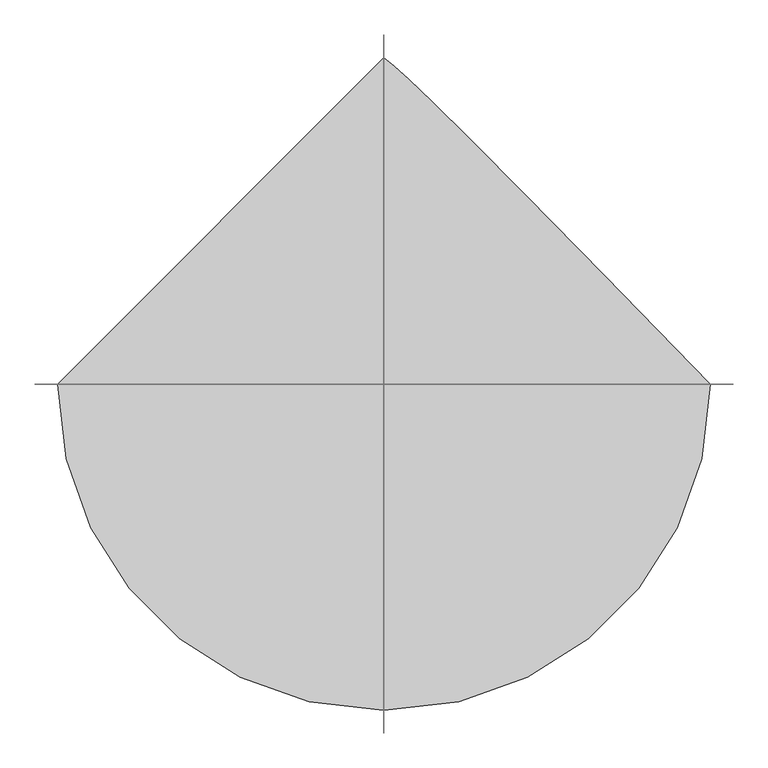
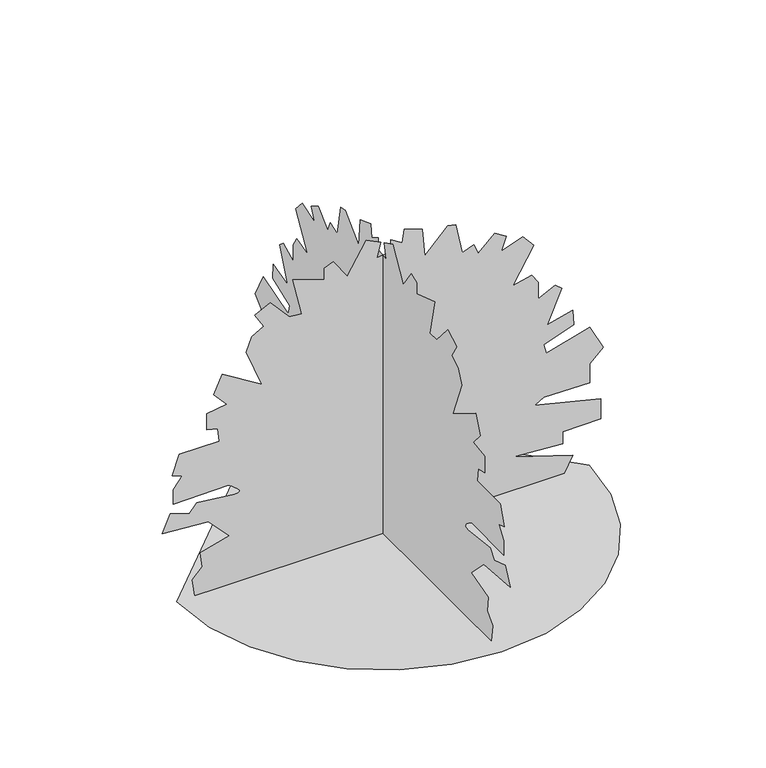
"""IFC4 building model written with IfcOpenShell, lengths in millimetres: proxy geometry, privet 26761 : privet 26761."""

import ifcopenshell
import ifcopenshell.guid

model = None  # the IFC model being written
_history = None  # IfcOwnerHistory: only IFC2X3 demands one
_inside = {}  # id of a spatial element -> (the spatial element, [elements in it])
_under = {}  # id of a project, library or spatial element -> (it, [spatial elements below it])
_declared = {}  # id of a project -> (the project, [libraries it declares])
_typed = {}  # id of a type object -> (the type object, [elements of that type])
_made_of = {}  # id of a material, layer set ... -> (it, [elements and type objects made of it])


def new_model(schema):
    """Start an empty IFC model of exactly this schema.

    Asked for "IFC4X3", IfcOpenShell would pick the latest addendum, in which some entities
    have other attributes; the version numbers below select the first issue.
    IFC2X3 requires an IfcOwnerHistory on every rooted entity: one is made here for all.
    """
    global model, _history
    if schema == "IFC4X3":
        model = ifcopenshell.file(schema_version=(4, 3, 0, 0))
    else:
        model = ifcopenshell.file(schema=schema)
    _inside.clear()
    _under.clear()
    _declared.clear()
    _typed.clear()
    _made_of.clear()
    _history = None
    if model.schema == "IFC2X3":
        org = make("IfcOrganization", Name="unknown")
        user = make(
            "IfcPersonAndOrganization",
            ThePerson=make("IfcPerson", FamilyName="unknown"),
            TheOrganization=org,
        )
        app = make(
            "IfcApplication",
            ApplicationDeveloper=org,
            Version="unknown",
            ApplicationFullName="unknown",
            ApplicationIdentifier="unknown",
        )
        _history = make(
            "IfcOwnerHistory",
            OwningUser=user,
            OwningApplication=app,
            ChangeAction="ADDED",
            CreationDate=0,
        )
    return model


def make(cls, **values):
    """One entity of the class cls with the attributes given. An attribute that is None is left unset."""
    return model.create_entity(
        cls, **{name: value for name, value in values.items() if value is not None}
    )


def rooted(cls, **values):
    """An entity with a GlobalId (a new one), such as an element, a storey or a relation."""
    return make(cls, GlobalId=ifcopenshell.guid.new(), OwnerHistory=_history, **values)


def si_unit(unit_type, name, prefix=None):
    """IfcSIUnit, for example si_unit("LENGTHUNIT", "METRE", prefix="MILLI")."""
    return make("IfcSIUnit", UnitType=unit_type, Prefix=prefix, Name=name)


def assignment(units):
    """IfcUnitAssignment: the units of a project."""
    return None if units is None else make("IfcUnitAssignment", Units=units)


def point(xyz):
    """IfcCartesianPoint."""
    return None if xyz is None else make("IfcCartesianPoint", Coordinates=xyz)


def direction(xyz):
    """IfcDirection."""
    return None if xyz is None else make("IfcDirection", DirectionRatios=xyz)


def frame(location, z_axis=None, x_axis=None):
    """IfcAxis2Placement3D, a coordinate frame: its origin and axes. An axis left out is left unset."""
    return make(
        "IfcAxis2Placement3D",
        Location=point(location),
        Axis=direction(z_axis),
        RefDirection=direction(x_axis),
    )


def origin():
    """The frame at (0, 0, 0) with its axes left unset."""
    return frame((0.0, 0.0, 0.0))


def place(relative_to, where):
    """IfcLocalPlacement: puts the frame where relative to a parent placement (None: the world)."""
    return make(
        "IfcLocalPlacement", PlacementRelTo=relative_to, RelativePlacement=where
    )


def context(
    kind, dimensions, precision=None, world=None, true_north=None, identifier=None
):
    """IfcGeometricRepresentationContext, for example the 3D "Model" context."""
    return make(
        "IfcGeometricRepresentationContext",
        ContextIdentifier=identifier,
        ContextType=kind,
        CoordinateSpaceDimension=dimensions,
        Precision=precision,
        WorldCoordinateSystem=world,
        TrueNorth=true_north,
    )


def project(units=None, contexts=None):
    """IfcProject with its units and contexts."""
    return rooted(
        "IfcProject",
        Name="project",
        RepresentationContexts=contexts,
        UnitsInContext=assignment(units),
    )


def spatial(cls, under=None, at=None, **own):
    """A site, building, storey or space (cls), placed at a placement, below another one or the project."""
    s = rooted(cls, ObjectPlacement=at, **own)
    if under is not None:
        _under.setdefault(under.id(), (under, []))[1].append(s)
    return s


def point_list(points):
    """IfcCartesianPointList2D or 3D."""
    cls = (
        "IfcCartesianPointList2D" if len(points[0]) == 2 else "IfcCartesianPointList3D"
    )
    return make(cls, CoordList=points)


def triangles(points, corners, closed=None, point_numbers=None):
    """IfcTriangulatedFaceSet: each triangle names its three corners, points numbered from 1."""
    return make(
        "IfcTriangulatedFaceSet",
        Coordinates=point_list(points),
        Closed=closed,
        CoordIndex=corners,
        PnIndex=point_numbers,
    )


def shape(context_of_items, identifier, shape_type, items):
    """IfcShapeRepresentation: the items that make up one representation, for example the "Body"."""
    return make(
        "IfcShapeRepresentation",
        ContextOfItems=context_of_items,
        RepresentationIdentifier=identifier,
        RepresentationType=shape_type,
        Items=items,
    )


def source(mapping_origin, context_of_items, identifier, shape_type, items):
    """IfcRepresentationMap: a shape defined once, which mapped items show again and again."""
    return make(
        "IfcRepresentationMap",
        MappingOrigin=mapping_origin,
        MappedRepresentation=shape(context_of_items, identifier, shape_type, items),
    )


def transform(
    local_origin,
    x_axis=None,
    y_axis=None,
    z_axis=None,
    scale=None,
    scale2=None,
    scale3=None,
    uniform=True,
):
    """IfcCartesianTransformationOperator3D, or its non-uniform kind. x_axis, y_axis, z_axis: its Axis1, 2, 3."""
    if uniform:
        return make(
            "IfcCartesianTransformationOperator3D",
            Axis1=direction(x_axis),
            Axis2=direction(y_axis),
            LocalOrigin=point(local_origin),
            Scale=scale,
            Axis3=direction(z_axis),
        )
    return make(
        "IfcCartesianTransformationOperator3DnonUniform",
        Axis1=direction(x_axis),
        Axis2=direction(y_axis),
        LocalOrigin=point(local_origin),
        Scale=scale,
        Axis3=direction(z_axis),
        Scale2=scale2,
        Scale3=scale3,
    )


def mapped(mapping_source, mapping_target):
    """IfcMappedItem: shows the shape of a source again, moved by a transform."""
    return make(
        "IfcMappedItem", MappingSource=mapping_source, MappingTarget=mapping_target
    )


def made_of(thing, what):
    """Note that an element or type object is made of a material, layer set ...; save() writes the relation."""
    if what is not None:
        _made_of.setdefault(what.id(), (what, []))[1].append(thing)
    return thing


def element(
    cls,
    number,
    at=None,
    inside=None,
    cuts=None,
    type_object=None,
    material=None,
    context=None,
    identifier="Body",
    shape_type=None,
    held_by="IfcProductDefinitionShape",
    body=None,
    shapes=None,
    **own,
):
    """One element of the class cls, such as IfcWall. Its Tag is "e" and its number.

    at: its placement. inside: the storey or other place that contains it. cuts: it is an
    opening in that element (IfcRelVoidsElement). A single representation is given by context,
    identifier, shape_type and body (its items); several are given by shapes. held_by: the class
    of the entity that holds the representations. save() writes the other relations.
    """
    e = rooted(cls, Tag="e%d" % number, ObjectPlacement=at, **own)
    if body is not None:
        shapes = [shape(context, identifier, shape_type, body)]
    if shapes is not None:
        e.Representation = make(held_by, Representations=shapes)
    if inside is not None:
        _inside.setdefault(inside.id(), (inside, []))[1].append(e)
    if cuts is not None:
        rooted(
            "IfcRelVoidsElement", RelatingBuildingElement=cuts, RelatedOpeningElement=e
        )
    if type_object is not None:
        _typed.setdefault(type_object.id(), (type_object, []))[1].append(e)
    return made_of(e, material)


def aggregate(whole, parts):
    """IfcRelAggregates: a whole, such as a stair, and the parts it consists of."""
    return rooted("IfcRelAggregates", RelatingObject=whole, RelatedObjects=parts)


def save(model, path):
    """Write the relations noted so far, then the file.

    IfcRelAggregates (storeys below a building ...), IfcRelContainedInSpatialStructure (elements
    in a storey), IfcRelDefinesByType, IfcRelAssociatesMaterial and IfcRelDeclares: one each for
    every whole, place, type object, material and project.
    """
    for whole, parts in _under.values():
        aggregate(whole, parts)
    for where, things in _inside.values():
        rooted(
            "IfcRelContainedInSpatialStructure",
            RelatedElements=things,
            RelatingStructure=where,
        )
    for kind, things in _typed.values():
        rooted("IfcRelDefinesByType", RelatedObjects=things, RelatingType=kind)
    for what, things in _made_of.values():
        rooted("IfcRelAssociatesMaterial", RelatedObjects=things, RelatingMaterial=what)
    for by, libraries in _declared.values():
        rooted("IfcRelDeclares", RelatingContext=by, RelatedDefinitions=libraries)
    model.write(path)


def entourage_76426c84(model_context):
    return source(origin(), model_context, "Body", "Tessellation", [
        triangles([(-629.6484856, 0.0, 4.95e-05), (-613.003862, -144.2738427, 4.95e-05), (-565.5947282, -276.766137, 4.95e-05), (-491.2235046, -393.6824018, 4.95e-05), (-393.6824018, -491.2235046, 4.95e-05), (-276.766137, -565.5947282, 4.95e-05), (-144.2738427, -613.003862, 4.95e-05), (2.75e-05, -629.6484856, 4.95e-05), (144.2738427, -613.003862, 4.95e-05), (276.766137, -565.5947282, 4.95e-05), (393.6824018, -491.2235046, 4.95e-05), (491.2235046, -393.6824018, 4.95e-05), (565.5947282, -276.766137, 4.95e-05), (613.003862, -144.2738427, 4.95e-05), (629.6484856, 5.5e-05, 4.95e-05), (425.0259828, 209.8919668, 4.95e-05), (273.329519, 364.4266657, 4.95e-05), (165.7386299, 472.8288062, 4.95e-05), (93.4306343, 544.3247692, 4.95e-05), (47.5853949, 588.1448779, 4.95e-05), (19.3822403, 613.5093544, 4.95e-05), (-8.26e-05, 629.6484856, 4.95e-05), (-2.3e-06, -573.7887774, 0.0), (-2.3e-06, -582.0844193, 55.3049682), (-2.3e-06, -551.6679256, 85.7227472), (-2.3e-06, -557.1974936, 132.7320781), (0.0, -468.7089269, 157.747784), (0.0, -532.310568, 224.1137004), (0.0, -673.33906, 235.174635), (0.0, -648.4495909, 290.4795987), (0.0, -590.3800612, 271.1222591), (0.0, -568.2592094, 298.7752406), (0.0, -452.1176431, 284.9500125), (0.0, -441.363285, 285.9964966), (0.0, -436.849716, 288.9327454), (0.0, -437.5355026, 293.4387022), (0.0, -442.379284, 299.2019587), (0.0, -450.3447135, 305.9101067), (0.0, -460.3904303, 313.2456327), (0.0, -471.4750008, 320.898654), (0.0, -640.153949, 318.1325801), (0.0, -640.153949, 365.1403939), (0.0, -612.5034565, 401.0890354), (0.0, -642.9199865, 412.1507512), (0.0, -620.7990984, 472.9863184), (0.0, -499.1280004, 472.9863184), (0.0, -504.6575684, 514.4645279), (0.0, -537.840136, 522.7601698), (0.0, -537.840136, 575.3000951), (0.0, -477.0045688, 583.595737), (0.0, -515.7192842, 627.8400204), (0.0, -490.8323585, 685.9095137), (0.0, -369.1612241, 611.2487366), (0.0, -416.1690016, 730.1537607), (0.0, -399.5777178, 774.3980804), (0.0, -363.6291126, 796.521512), (0.0, -391.2820759, 840.7632156), (0.0, -344.2742984, 865.6526848), (0.0, -286.2022435, 799.2850061), (0.0, -247.4898354, 796.521512), (0.0, -275.1430711, 915.4265362), (0.0, -178.3586263, 882.2439686), (0.0, -178.3586263, 918.190103), (0.0, -150.7061354, 929.2517824), (0.0, -109.2271628, 868.4161789), (0.0, -51.1571472, 965.2003876), (0.0, -6.9130699, 943.0795721), (0.0, -17.9741141, 896.0692148), (0.0, 23.5046359, 901.5988192), (0.0, 23.5046359, 940.3134619), (0.0, 59.4527891, 918.190103), (0.0, 64.9833881, 959.6708559), (0.0, 120.2883518, 940.3134619), (0.0, 128.5842571, 851.8248951), (0.0, 197.7154571, 923.7221781), (0.0, 222.6026553, 918.190103), (0.0, 241.9594862, 821.4084377), (0.0, 277.9066016, 835.2336113), (0.0, 291.7343731, 802.0510437), (0.0, 341.5082245, 849.0588575), (0.0, 377.456866, 826.9379694), (0.0, 360.8655822, 785.4597599), (0.0, 427.2307174, 807.580648), (0.0, 460.413285, 768.8684761), (0.0, 396.8142237, 661.022588), (0.0, 454.883717, 674.8503777), (0.0, 474.2410747, 644.4313042), (0.0, 474.2410747, 591.8913789), (0.0, 526.7809999, 616.7782682), (0.0, 546.1357779, 600.1870208), (0.0, 501.8915308, 497.8732441), (0.0, 579.3183818, 517.2305655), (0.0, 582.0844193, 470.2202445), (0.0, 490.8323585, 437.0376769), (0.0, 499.1280004, 406.6211469), (0.0, 631.8583071, 445.3333188), (0.0, 673.33906, 365.1403939), (0.0, 631.8583071, 326.428222), (0.0, 631.8583071, 265.592673), (0.0, 490.8323585, 268.3587287), (0.0, 463.1793589, 251.7661732), (0.0, 665.0434181, 201.9918131), (0.0, 665.0434181, 138.3909441), (0.0, 548.9018517, 135.6256423), (0.0, 548.9018517, 96.9122169), (0.0, 399.5777178, 107.9731605), (0.0, 579.3183818, 49.9031495), (0.0, 554.4314198, 0.1285451), (-573.7887774, 9.96e-05, 4.86e-05), (-582.0844193, 9.63e-05, 55.3049682), (-551.6679256, 9.44e-05, 85.7227472), (-557.1974936, 9.16e-05, 132.7320781), (-468.7089269, 8.79e-05, 157.747784), (-532.310568, 8.39e-05, 224.1137004), (-673.33906, 8.33e-05, 235.174635), (-648.4495909, 8e-05, 290.4795987), (-590.3800612, 8.11e-05, 271.1222591), (-568.2592094, 7.95e-05, 298.7752406), (-452.1176431, 8.03e-05, 284.9500125), (-441.363285, 8.02e-05, 285.9964966), (-436.849716, 8.01e-05, 288.9327454), (-437.5355026, 7.98e-05, 293.4387022), (-442.379284, 7.95e-05, 299.2019587), (-450.3447135, 7.91e-05, 305.9101067), (-460.3904303, 7.86e-05, 313.2456327), (-471.4750008, 7.82e-05, 320.898654), (-640.153949, 7.83e-05, 318.1325801), (-640.153949, 7.55e-05, 365.1403939), (-612.5034565, 7.34e-05, 401.0890354), (-642.9199865, 7.27e-05, 412.1507512), (-620.7990984, 6.91e-05, 472.9863184), (-499.1280004, 6.91e-05, 472.9863184), (-504.6575684, 6.66e-05, 514.4645279), (-537.840136, 6.61e-05, 522.7601698), (-537.840136, 6.3e-05, 575.3000951), (-477.0045688, 6.25e-05, 583.595737), (-515.7192842, 5.99e-05, 627.8400204), (-490.8323585, 5.64e-05, 685.9095137), (-369.1612241, 6.09e-05, 611.2487366), (-416.1690016, 5.38e-05, 730.1537607), (-399.5777178, 5.11e-05, 774.3980804), (-363.6291126, 4.98e-05, 796.521512), (-391.2820759, 4.72e-05, 840.7632156), (-344.2742984, 4.57e-05, 865.6526848), (-286.2022435, 4.96e-05, 799.2850061), (-247.4898354, 4.98e-05, 796.521512), (-275.1430711, 4.27e-05, 915.4265362), (-178.3586263, 4.47e-05, 882.2439686), (-178.3586263, 4.26e-05, 918.190103), (-150.7061354, 4.19e-05, 929.2517824), (-109.2274081, 4.55e-05, 868.4161789), (-51.1571472, 3.98e-05, 965.2003876), (-6.9131466, 4.11e-05, 943.0795721), (-17.9741902, 4.39e-05, 896.0692148), (23.5045859, 4.35e-05, 901.5988192), (23.5045859, 4.12e-05, 940.3134619), (59.4527891, 4.26e-05, 918.190103), (64.9833881, 4.01e-05, 959.6708559), (120.2883518, 4.12e-05, 940.3134619), (128.5840028, 4.65e-05, 851.8248951), (197.7152028, 4.22e-05, 923.7221781), (222.6026553, 4.26e-05, 918.190103), (241.9592318, 4.83e-05, 821.4084377), (277.9066016, 4.75e-05, 835.2336113), (291.7343731, 4.95e-05, 802.0510437), (341.5082245, 4.67e-05, 849.0588575), (377.456866, 4.8e-05, 826.9379694), (360.8655822, 5.05e-05, 785.4597599), (427.2307174, 4.92e-05, 807.580648), (460.413285, 5.15e-05, 768.8684761), (396.8142237, 5.79e-05, 661.022588), (454.883717, 5.71e-05, 674.8503777), (474.2410747, 5.89e-05, 644.4313042), (474.2410747, 6.2e-05, 591.8913789), (526.7809999, 6.05e-05, 616.7782682), (546.1357779, 6.15e-05, 600.1870208), (501.8915308, 6.76e-05, 497.8732441), (579.3183818, 6.65e-05, 517.2305655), (582.0844193, 6.93e-05, 470.2202445), (490.8323585, 7.12e-05, 437.0376769), (499.1280004, 7.31e-05, 406.6211469), (631.8583071, 7.07e-05, 445.3333188), (673.33906, 7.55e-05, 365.1403939), (631.8583071, 7.78e-05, 326.428222), (631.8583071, 8.15e-05, 265.592673), (490.8323585, 8.13e-05, 268.3587287), (463.1793589, 8.23e-05, 251.7661732), (665.0434181, 8.52e-05, 201.9918131), (665.0434181, 8.9e-05, 138.3909441), (548.9018517, 8.92e-05, 135.6258967), (548.9018517, 9.15e-05, 96.9122169), (399.5777178, 9.09e-05, 107.9734149), (579.3183818, 9.43e-05, 49.9031495), (554.4314198, 9.73e-05, 0.1285937)], [[21, 22, 1], [20, 21, 1], [19, 20, 1], [18, 19, 1], [17, 18, 1], [17, 1, 2], [17, 2, 3], [17, 3, 4], [16, 17, 4], [16, 4, 5], [16, 5, 6], [16, 6, 7], [16, 7, 8], [16, 8, 9], [16, 9, 10], [16, 10, 11], [16, 11, 12], [15, 16, 12], [14, 15, 12], [13, 14, 12], [60, 61, 62], [69, 70, 71], [28, 29, 30], [28, 30, 31], [71, 72, 73], [71, 73, 74], [91, 92, 93], [91, 93, 94], [106, 107, 108], [106, 108, 23], [51, 52, 53], [50, 51, 53], [104, 105, 106], [56, 57, 58], [56, 58, 59], [98, 99, 100], [40, 41, 42], [40, 42, 43], [43, 44, 45], [43, 45, 46], [40, 43, 46], [28, 31, 32], [102, 103, 104], [101, 102, 104], [101, 104, 106], [77, 78, 79], [106, 23, 24], [106, 24, 25], [65, 66, 67], [65, 67, 68], [106, 25, 26], [106, 26, 27], [48, 49, 50], [47, 48, 50], [80, 81, 82], [79, 80, 82], [95, 96, 97], [95, 97, 98], [95, 98, 100], [63, 64, 65], [62, 63, 65], [89, 90, 91], [88, 89, 91], [27, 28, 32], [27, 32, 33], [106, 27, 33], [106, 33, 34], [106, 34, 35], [101, 106, 35], [101, 35, 36], [83, 84, 85], [82, 83, 85], [85, 86, 87], [85, 87, 88], [69, 71, 74], [75, 76, 77], [74, 75, 77], [60, 62, 65], [79, 82, 85], [95, 100, 101], [95, 101, 36], [94, 95, 36], [91, 94, 36], [88, 91, 36], [85, 88, 36], [79, 85, 36], [77, 79, 36], [74, 77, 36], [69, 74, 36], [68, 69, 36], [65, 68, 36], [60, 65, 36], [60, 36, 37], [60, 37, 38], [59, 60, 38], [59, 38, 39], [59, 39, 40], [47, 50, 53], [46, 47, 53], [40, 46, 53], [59, 40, 53], [59, 53, 54], [56, 59, 54], [56, 54, 55], [146, 147, 148], [155, 156, 157], [114, 115, 116], [114, 116, 117], [157, 158, 159], [157, 159, 160], [177, 178, 179], [177, 179, 180], [192, 193, 194], [192, 194, 109], [137, 138, 139], [136, 137, 139], [190, 191, 192], [142, 143, 144], [142, 144, 145], [184, 185, 186], [126, 127, 128], [126, 128, 129], [129, 130, 131], [129, 131, 132], [126, 129, 132], [114, 117, 118], [188, 189, 190], [187, 188, 190], [187, 190, 192], [163, 164, 165], [192, 109, 110], [192, 110, 111], [151, 152, 153], [151, 153, 154], [192, 111, 112], [192, 112, 113], [134, 135, 136], [133, 134, 136], [166, 167, 168], [165, 166, 168], [181, 182, 183], [181, 183, 184], [181, 184, 186], [149, 150, 151], [148, 149, 151], [175, 176, 177], [174, 175, 177], [113, 114, 118], [113, 118, 119], [192, 113, 119], [192, 119, 120], [192, 120, 121], [187, 192, 121], [187, 121, 122], [169, 170, 171], [168, 169, 171], [171, 172, 173], [171, 173, 174], [155, 157, 160], [161, 162, 163], [160, 161, 163], [146, 148, 151], [165, 168, 171], [181, 186, 187], [181, 187, 122], [180, 181, 122], [177, 180, 122], [174, 177, 122], [171, 174, 122], [165, 171, 122], [163, 165, 122], [160, 163, 122], [155, 160, 122], [154, 155, 122], [151, 154, 122], [146, 151, 122], [146, 122, 123], [146, 123, 124], [145, 146, 124], [145, 124, 125], [145, 125, 126], [133, 136, 139], [132, 133, 139], [126, 132, 139], [145, 126, 139], [145, 139, 140], [142, 145, 140], [142, 140, 141]], closed=False),
    ])


if __name__ == "__main__":
    model = new_model("IFC4")
    model_context = context("Model", 3, world=origin())
    ifc_project = project(units=[si_unit("LENGTHUNIT", "METRE", prefix="MILLI")], contexts=[model_context])
    site = spatial("IfcSite", under=ifc_project)
    building = spatial("IfcBuilding", under=site)
    placement = place(None, origin())
    entourage_shape = entourage_76426c84(model_context)
    element("IfcBuildingElementProxy", 1, Name="privet 26761 : privet 26761", ObjectType="privet 26761 : privet 26761", at=placement, inside=building, context=model_context, shape_type="MappedRepresentation", body=[
        mapped(entourage_shape, transform((0.0, 0.0, 0.0), x_axis=(1.0, 0.0, 0.0), y_axis=(0.0, 1.0, 0.0), z_axis=(0.0, 0.0, 1.0))),
    ])
    save(model, "model.ifc")

# Revit data of these elements
# Type "privet 26761 : privet 26761"
#   built-in parameter 1005195 = "RPC-16-FXGX-NJPX-PH0L-8000-ST1L-LVER-AU"
#   Height = 0
